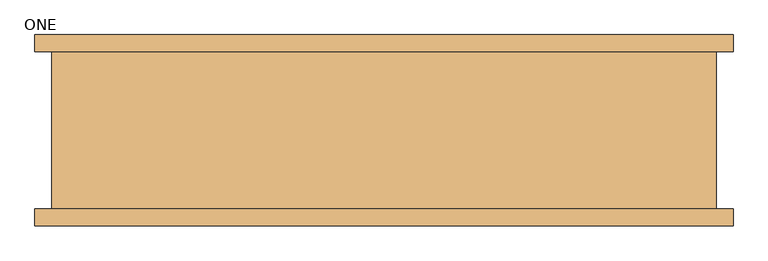
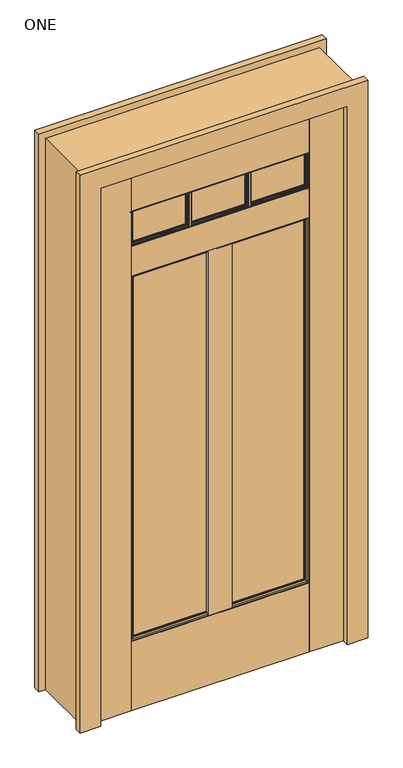
"""IFC4 building model written with IfcOpenShell, lengths in millimetres: door geometry, Door-Exterior-Simpson-Craftsman : ONE."""

from ifc_helpers import new_model, si_unit, point, frame, frame_2d, origin, origin_with_axes, place, context, project, spatial, polyline, circle_curve, ellipse_curve, trimmed, segment, composite_curve, outline, extrude, faceted_brep, source, transform, mapped, element, save
from ifc_brep_helpers import plane_surface, cylinder_surface, advanced_brep


def one_efa2d6c3(model_context):
    return source(origin(), model_context, "Body", "SolidModel", [
        extrude(outline(composite_curve([segment(polyline([(114.0354167, -78.5495), (114.0354167, -80.264), (116.1486027, -80.6366117)]), True, "CONTINUOUS"), segment(trimmed(circle_curve(frame_2d((115.7075363, -83.1380234)), 2.54), [point((116.1486027, -80.6366117))], [point((118.208948, -82.696957))], False, "CARTESIAN"), True, "CONTINUOUS"), segment(polyline([(118.208948, -82.696957), (118.7696182, -85.8766758), (120.0821906, -85.991511)]), True, "CONTINUOUS"), segment(trimmed(circle_curve(frame_2d((120.0157779, -86.7506113)), 0.762), [point((120.0821906, -85.991511))], [point((120.7662014, -86.6182914))], False, "CARTESIAN"), True, "CONTINUOUS"), segment(polyline([(120.7662014, -86.6182914), (121.1685282, -88.9), (98.9648051, -88.9), (99.3671319, -86.6182914)]), True, "CONTINUOUS"), segment(trimmed(circle_curve(frame_2d((100.1175554, -86.7506113)), 0.762), [point((99.3671319, -86.6182914))], [point((100.0511427, -85.991511))], False, "CARTESIAN"), True, "CONTINUOUS"), segment(polyline([(100.0511427, -85.991511), (101.3637152, -85.8766758), (101.9243854, -82.696957)]), True, "CONTINUOUS"), segment(trimmed(circle_curve(frame_2d((104.4257971, -83.1380234)), 2.54), [point((101.9243854, -82.696957))], [point((103.9847307, -80.6366117))], False, "CARTESIAN"), True, "CONTINUOUS"), segment(polyline([(103.9847307, -80.6366117), (106.0979167, -80.264), (106.0979167, -78.5495), (114.0354167, -78.5495)]), True, "CONTINUOUS")], self_intersect=False)), frame((0.0, 0.0, 1817.6875), z_axis=(0.0, 0.0, 1.0), x_axis=(1.0, 0.0, 0.0)), (0.0, 0.0, 1.0), 139.7),
        extrude(outline(composite_curve([segment(polyline([(114.0354167, -118.3005), (106.0979167, -118.3005), (106.0979167, -116.586), (103.9847307, -116.2133883)]), True, "CONTINUOUS"), segment(trimmed(circle_curve(frame_2d((104.4257971, -113.7119766)), 2.54), [point((103.9847307, -116.2133883))], [point((101.9243854, -114.153043))], False, "CARTESIAN"), True, "CONTINUOUS"), segment(polyline([(101.9243854, -114.153043), (101.3637152, -110.9733242), (100.0511427, -110.858489)]), True, "CONTINUOUS"), segment(trimmed(circle_curve(frame_2d((100.1175554, -110.0993887)), 0.762), [point((100.0511427, -110.858489))], [point((99.3671319, -110.2317086))], False, "CARTESIAN"), True, "CONTINUOUS"), segment(polyline([(99.3671319, -110.2317086), (98.9648051, -107.95), (121.1685282, -107.95), (120.7662014, -110.2317086)]), True, "CONTINUOUS"), segment(trimmed(circle_curve(frame_2d((120.0157779, -110.0993887)), 0.762), [point((120.7662014, -110.2317086))], [point((120.0821906, -110.858489))], False, "CARTESIAN"), True, "CONTINUOUS"), segment(polyline([(120.0821906, -110.858489), (118.7696182, -110.9733242), (118.208948, -114.153043)]), True, "CONTINUOUS"), segment(trimmed(circle_curve(frame_2d((115.7075363, -113.7119766)), 2.54), [point((118.208948, -114.153043))], [point((116.1486027, -116.2133883))], False, "CARTESIAN"), True, "CONTINUOUS"), segment(polyline([(116.1486027, -116.2133883), (114.0354167, -116.586), (114.0354167, -118.3005)]), True, "CONTINUOUS")], self_intersect=False)), frame((0.0, 0.0, 1817.6875), z_axis=(0.0, 0.0, 1.0), x_axis=(1.0, 0.0, 0.0)), (0.0, 0.0, 1.0), 139.7),
        extrude(outline(composite_curve([segment(polyline([(-106.0979167, -78.5495), (-106.0979167, -80.264), (-103.9847307, -80.6366117)]), True, "CONTINUOUS"), segment(trimmed(circle_curve(frame_2d((-104.4257971, -83.1380234)), 2.54), [point((-103.9847307, -80.6366117))], [point((-101.9243854, -82.696957))], False, "CARTESIAN"), True, "CONTINUOUS"), segment(polyline([(-101.9243854, -82.696957), (-101.3637152, -85.8766758), (-100.0511427, -85.991511)]), True, "CONTINUOUS"), segment(trimmed(circle_curve(frame_2d((-100.1175554, -86.7506113)), 0.762), [point((-100.0511427, -85.991511))], [point((-99.3671319, -86.6182914))], False, "CARTESIAN"), True, "CONTINUOUS"), segment(polyline([(-99.3671319, -86.6182914), (-98.9648051, -88.9), (-121.1685282, -88.9), (-120.7662014, -86.6182914)]), True, "CONTINUOUS"), segment(trimmed(circle_curve(frame_2d((-120.0157779, -86.7506113)), 0.762), [point((-120.7662014, -86.6182914))], [point((-120.0821906, -85.991511))], False, "CARTESIAN"), True, "CONTINUOUS"), segment(polyline([(-120.0821906, -85.991511), (-118.7696182, -85.8766758), (-118.208948, -82.696957)]), True, "CONTINUOUS"), segment(trimmed(circle_curve(frame_2d((-115.7075363, -83.1380234)), 2.54), [point((-118.208948, -82.696957))], [point((-116.1486027, -80.6366117))], False, "CARTESIAN"), True, "CONTINUOUS"), segment(polyline([(-116.1486027, -80.6366117), (-114.0354167, -80.264), (-114.0354167, -78.5495), (-106.0979167, -78.5495)]), True, "CONTINUOUS")], self_intersect=False)), frame((0.0, 0.0, 1817.6875), z_axis=(0.0, 0.0, 1.0), x_axis=(1.0, 0.0, 0.0)), (0.0, 0.0, 1.0), 139.7),
        extrude(outline(composite_curve([segment(polyline([(-106.0979167, -118.3005), (-114.0354167, -118.3005), (-114.0354167, -116.586), (-116.1486027, -116.2133883)]), True, "CONTINUOUS"), segment(trimmed(circle_curve(frame_2d((-115.7075363, -113.7119766)), 2.54), [point((-116.1486027, -116.2133883))], [point((-118.208948, -114.153043))], False, "CARTESIAN"), True, "CONTINUOUS"), segment(polyline([(-118.208948, -114.153043), (-118.7696182, -110.9733242), (-120.0821906, -110.858489)]), True, "CONTINUOUS"), segment(trimmed(circle_curve(frame_2d((-120.0157779, -110.0993887)), 0.762), [point((-120.0821906, -110.858489))], [point((-120.7662014, -110.2317086))], False, "CARTESIAN"), True, "CONTINUOUS"), segment(polyline([(-120.7662014, -110.2317086), (-121.1685282, -107.95), (-98.9648051, -107.95), (-99.3671319, -110.2317086)]), True, "CONTINUOUS"), segment(trimmed(circle_curve(frame_2d((-100.1175554, -110.0993887)), 0.762), [point((-99.3671319, -110.2317086))], [point((-100.0511427, -110.858489))], False, "CARTESIAN"), True, "CONTINUOUS"), segment(polyline([(-100.0511427, -110.858489), (-101.3637152, -110.9733242), (-101.9243854, -114.153043)]), True, "CONTINUOUS"), segment(trimmed(circle_curve(frame_2d((-104.4257971, -113.7119766)), 2.54), [point((-101.9243854, -114.153043))], [point((-103.9847307, -116.2133883))], False, "CARTESIAN"), True, "CONTINUOUS"), segment(polyline([(-103.9847307, -116.2133883), (-106.0979167, -116.586), (-106.0979167, -118.3005)]), True, "CONTINUOUS")], self_intersect=False)), frame((0.0, 0.0, 1817.6875), z_axis=(0.0, 0.0, 1.0), x_axis=(1.0, 0.0, 0.0)), (0.0, 0.0, 1.0), 139.7),
        extrude(outline(polyline([(44.45, -78.7796875), (44.45, -118.0703125), (-44.45, -118.0703125), (-44.45, -78.7796875), (44.45, -78.7796875)])), frame((0.0, 0.0, 271.4625), z_axis=(0.0, 0.0, 1.0), x_axis=(1.0, 0.0, 0.0)), (0.0, 0.0, 1.0), 1431.925),
        extrude(outline(polyline([(419.89375, -78.7796875), (419.89375, -118.0703125), (330.99375, -118.0703125), (330.99375, -78.7796875), (419.89375, -78.7796875)])), frame((0.0, 0.0, 271.4625), z_axis=(0.0, 0.0, 1.0), x_axis=(1.0, 0.0, 0.0)), (0.0, 0.0, 1.0), 1431.925),
        extrude(outline(polyline([(-330.99375, -78.7796875), (-330.99375, -118.0703125), (-419.89375, -118.0703125), (-419.89375, -78.7796875), (-330.99375, -78.7796875)])), frame((0.0, 0.0, 271.4625), z_axis=(0.0, 0.0, 1.0), x_axis=(1.0, 0.0, 0.0)), (0.0, 0.0, 1.0), 1431.925),
        extrude(outline(polyline([(330.2, -107.95), (-330.2, -107.95), (-330.2, -88.9), (330.2, -88.9), (330.2, -107.95)])), frame((0.0, 0.0, 271.4625), z_axis=(0.0, 0.0, 1.0), x_axis=(1.0, 0.0, 0.0)), (0.0, 0.0, 1.0), 1431.925),
        extrude(outline(composite_curve([segment(polyline([(334.16875, -78.5495), (334.16875, -80.264), (336.281936, -80.6366117)]), True, "CONTINUOUS"), segment(trimmed(circle_curve(frame_2d((335.8408696, -83.1380234)), 2.54), [point((336.281936, -80.6366117))], [point((338.3422813, -82.696957))], False, "CARTESIAN"), True, "CONTINUOUS"), segment(polyline([(338.3422813, -82.696957), (338.9029515, -85.8766758), (340.2155239, -85.991511)]), True, "CONTINUOUS"), segment(trimmed(circle_curve(frame_2d((340.1491113, -86.7506113)), 0.762), [point((340.2155239, -85.991511))], [point((340.8995348, -86.6182914))], False, "CARTESIAN"), True, "CONTINUOUS"), segment(polyline([(340.8995348, -86.6182914), (341.3018616, -88.9), (319.0981384, -88.9), (319.5004652, -86.6182914)]), True, "CONTINUOUS"), segment(trimmed(circle_curve(frame_2d((320.2508887, -86.7506113)), 0.762), [point((319.5004652, -86.6182914))], [point((320.1844761, -85.991511))], False, "CARTESIAN"), True, "CONTINUOUS"), segment(polyline([(320.1844761, -85.991511), (321.4970485, -85.8766758), (322.0577187, -82.696957)]), True, "CONTINUOUS"), segment(trimmed(circle_curve(frame_2d((324.5591304, -83.1380234)), 2.54), [point((322.0577187, -82.696957))], [point((324.118064, -80.6366117))], False, "CARTESIAN"), True, "CONTINUOUS"), segment(polyline([(324.118064, -80.6366117), (326.23125, -80.264), (326.23125, -78.5495), (334.16875, -78.5495)]), True, "CONTINUOUS")], self_intersect=False)), frame((0.0, 0.0, 1817.6875), z_axis=(0.0, 0.0, 1.0), x_axis=(1.0, 0.0, 0.0)), (0.0, 0.0, 1.0), 139.7),
        extrude(outline(composite_curve([segment(polyline([(334.16875, -118.3005), (326.23125, -118.3005), (326.23125, -116.586), (324.118064, -116.2133883)]), True, "CONTINUOUS"), segment(trimmed(circle_curve(frame_2d((324.5591304, -113.7119766)), 2.54), [point((324.118064, -116.2133883))], [point((322.0577187, -114.153043))], False, "CARTESIAN"), True, "CONTINUOUS"), segment(polyline([(322.0577187, -114.153043), (321.4970485, -110.9733242), (320.1844761, -110.858489)]), True, "CONTINUOUS"), segment(trimmed(circle_curve(frame_2d((320.2508887, -110.0993887)), 0.762), [point((320.1844761, -110.858489))], [point((319.5004652, -110.2317086))], False, "CARTESIAN"), True, "CONTINUOUS"), segment(polyline([(319.5004652, -110.2317086), (319.0981384, -107.95), (341.3018616, -107.95), (340.8995348, -110.2317086)]), True, "CONTINUOUS"), segment(trimmed(circle_curve(frame_2d((340.1491113, -110.0993887)), 0.762), [point((340.8995348, -110.2317086))], [point((340.2155239, -110.858489))], False, "CARTESIAN"), True, "CONTINUOUS"), segment(polyline([(340.2155239, -110.858489), (338.9029515, -110.9733242), (338.3422813, -114.153043)]), True, "CONTINUOUS"), segment(trimmed(circle_curve(frame_2d((335.8408696, -113.7119766)), 2.54), [point((338.3422813, -114.153043))], [point((336.281936, -116.2133883))], False, "CARTESIAN"), True, "CONTINUOUS"), segment(polyline([(336.281936, -116.2133883), (334.16875, -116.586), (334.16875, -118.3005)]), True, "CONTINUOUS")], self_intersect=False)), frame((0.0, 0.0, 1817.6875), z_axis=(0.0, 0.0, 1.0), x_axis=(1.0, 0.0, 0.0)), (0.0, 0.0, 1.0), 139.7),
        extrude(outline(composite_curve([segment(polyline([(-78.5495, 1813.71875), (-80.264, 1813.71875), (-80.6366117, 1811.605564)]), True, "CONTINUOUS"), segment(trimmed(circle_curve(frame_2d((-83.1380234, 1812.0466304)), 2.54), [point((-80.6366117, 1811.605564))], [point((-82.696957, 1809.5452187))], False, "CARTESIAN"), True, "CONTINUOUS"), segment(polyline([(-82.696957, 1809.5452187), (-85.8766758, 1808.9845485), (-85.991511, 1807.6719761)]), True, "CONTINUOUS"), segment(trimmed(circle_curve(frame_2d((-86.7506113, 1807.7383887)), 0.762), [point((-85.991511, 1807.6719761))], [point((-86.6182914, 1806.9879652))], False, "CARTESIAN"), True, "CONTINUOUS"), segment(polyline([(-86.6182914, 1806.9879652), (-88.9, 1806.5856384), (-88.9, 1828.7893616), (-86.6182914, 1828.3870348)]), True, "CONTINUOUS"), segment(trimmed(circle_curve(frame_2d((-86.7506113, 1827.6366113)), 0.762), [point((-86.6182914, 1828.3870348))], [point((-85.991511, 1827.7030239))], False, "CARTESIAN"), True, "CONTINUOUS"), segment(polyline([(-85.991511, 1827.7030239), (-85.8766758, 1826.3904515), (-82.696957, 1825.8297813)]), True, "CONTINUOUS"), segment(trimmed(circle_curve(frame_2d((-83.1380234, 1823.3283696)), 2.54), [point((-82.696957, 1825.8297813))], [point((-80.6366117, 1823.769436))], False, "CARTESIAN"), True, "CONTINUOUS"), segment(polyline([(-80.6366117, 1823.769436), (-80.264, 1821.65625), (-78.5495, 1821.65625), (-78.5495, 1813.71875)]), True, "CONTINUOUS")], self_intersect=False)), frame((-330.2, 0.0, 0.0), z_axis=(1.0, 0.0, 0.0), x_axis=(0.0, 1.0, 0.0)), (0.0, 0.0, 1.0), 660.4),
        extrude(outline(composite_curve([segment(polyline([(-118.3005, 1813.71875), (-118.3005, 1821.65625), (-116.586, 1821.65625), (-116.2133883, 1823.769436)]), True, "CONTINUOUS"), segment(trimmed(circle_curve(frame_2d((-113.7119766, 1823.3283696)), 2.54), [point((-116.2133883, 1823.769436))], [point((-114.153043, 1825.8297813))], False, "CARTESIAN"), True, "CONTINUOUS"), segment(polyline([(-114.153043, 1825.8297813), (-110.9733242, 1826.3904515), (-110.858489, 1827.7030239)]), True, "CONTINUOUS"), segment(trimmed(circle_curve(frame_2d((-110.0993887, 1827.6366113)), 0.762), [point((-110.858489, 1827.7030239))], [point((-110.2317086, 1828.3870348))], False, "CARTESIAN"), True, "CONTINUOUS"), segment(polyline([(-110.2317086, 1828.3870348), (-107.95, 1828.7893616), (-107.95, 1806.5856384), (-110.2317086, 1806.9879652)]), True, "CONTINUOUS"), segment(trimmed(circle_curve(frame_2d((-110.0993887, 1807.7383887)), 0.762), [point((-110.2317086, 1806.9879652))], [point((-110.858489, 1807.6719761))], False, "CARTESIAN"), True, "CONTINUOUS"), segment(polyline([(-110.858489, 1807.6719761), (-110.9733242, 1808.9845485), (-114.153043, 1809.5452187)]), True, "CONTINUOUS"), segment(trimmed(circle_curve(frame_2d((-113.7119766, 1812.0466304)), 2.54), [point((-114.153043, 1809.5452187))], [point((-116.2133883, 1811.605564))], False, "CARTESIAN"), True, "CONTINUOUS"), segment(polyline([(-116.2133883, 1811.605564), (-116.586, 1813.71875), (-118.3005, 1813.71875)]), True, "CONTINUOUS")], self_intersect=False)), frame((-330.2, 0.0, 0.0), z_axis=(1.0, 0.0, 0.0), x_axis=(0.0, 1.0, 0.0)), (0.0, 0.0, 1.0), 660.4),
        extrude(outline(composite_curve([segment(polyline([(-78.5495, 1953.41875), (-80.264, 1953.41875), (-80.6366117, 1951.305564)]), True, "CONTINUOUS"), segment(trimmed(circle_curve(frame_2d((-83.1380234, 1951.7466304)), 2.54), [point((-80.6366117, 1951.305564))], [point((-82.696957, 1949.2452187))], False, "CARTESIAN"), True, "CONTINUOUS"), segment(polyline([(-82.696957, 1949.2452187), (-85.8766758, 1948.6845485), (-85.991511, 1947.3719761)]), True, "CONTINUOUS"), segment(trimmed(circle_curve(frame_2d((-86.7506113, 1947.4383887)), 0.762), [point((-85.991511, 1947.3719761))], [point((-86.6182914, 1946.6879652))], False, "CARTESIAN"), True, "CONTINUOUS"), segment(polyline([(-86.6182914, 1946.6879652), (-88.9, 1946.2856384), (-88.9, 1968.4893616), (-86.6182914, 1968.0870348)]), True, "CONTINUOUS"), segment(trimmed(circle_curve(frame_2d((-86.7506113, 1967.3366113)), 0.762), [point((-86.6182914, 1968.0870348))], [point((-85.991511, 1967.4030239))], False, "CARTESIAN"), True, "CONTINUOUS"), segment(polyline([(-85.991511, 1967.4030239), (-85.8766758, 1966.0904515), (-82.696957, 1965.5297813)]), True, "CONTINUOUS"), segment(trimmed(circle_curve(frame_2d((-83.1380234, 1963.0283696)), 2.54), [point((-82.696957, 1965.5297813))], [point((-80.6366117, 1963.469436))], False, "CARTESIAN"), True, "CONTINUOUS"), segment(polyline([(-80.6366117, 1963.469436), (-80.264, 1961.35625), (-78.5495, 1961.35625), (-78.5495, 1953.41875)]), True, "CONTINUOUS")], self_intersect=False)), frame((-330.2, 0.0, 0.0), z_axis=(1.0, 0.0, 0.0), x_axis=(0.0, 1.0, 0.0)), (0.0, 0.0, 1.0), 660.4),
        extrude(outline(composite_curve([segment(polyline([(-118.3005, 1953.41875), (-118.3005, 1961.35625), (-116.586, 1961.35625), (-116.2133883, 1963.469436)]), True, "CONTINUOUS"), segment(trimmed(circle_curve(frame_2d((-113.7119766, 1963.0283696)), 2.54), [point((-116.2133883, 1963.469436))], [point((-114.153043, 1965.5297813))], False, "CARTESIAN"), True, "CONTINUOUS"), segment(polyline([(-114.153043, 1965.5297813), (-110.9733242, 1966.0904515), (-110.858489, 1967.4030239)]), True, "CONTINUOUS"), segment(trimmed(circle_curve(frame_2d((-110.0993887, 1967.3366113)), 0.762), [point((-110.858489, 1967.4030239))], [point((-110.2317086, 1968.0870348))], False, "CARTESIAN"), True, "CONTINUOUS"), segment(polyline([(-110.2317086, 1968.0870348), (-107.95, 1968.4893616), (-107.95, 1946.2856384), (-110.2317086, 1946.6879652)]), True, "CONTINUOUS"), segment(trimmed(circle_curve(frame_2d((-110.0993887, 1947.4383887)), 0.762), [point((-110.2317086, 1946.6879652))], [point((-110.858489, 1947.3719761))], False, "CARTESIAN"), True, "CONTINUOUS"), segment(polyline([(-110.858489, 1947.3719761), (-110.9733242, 1948.6845485), (-114.153043, 1949.2452187)]), True, "CONTINUOUS"), segment(trimmed(circle_curve(frame_2d((-113.7119766, 1951.7466304)), 2.54), [point((-114.153043, 1949.2452187))], [point((-116.2133883, 1951.305564))], False, "CARTESIAN"), True, "CONTINUOUS"), segment(polyline([(-116.2133883, 1951.305564), (-116.586, 1953.41875), (-118.3005, 1953.41875)]), True, "CONTINUOUS")], self_intersect=False)), frame((-330.2, 0.0, 0.0), z_axis=(1.0, 0.0, 0.0), x_axis=(0.0, 1.0, 0.0)), (0.0, 0.0, 1.0), 660.4),
        extrude(outline(composite_curve([segment(polyline([(-326.23125, -78.5495), (-326.23125, -80.264), (-324.118064, -80.6366117)]), True, "CONTINUOUS"), segment(trimmed(circle_curve(frame_2d((-324.5591304, -83.1380234)), 2.54), [point((-324.118064, -80.6366117))], [point((-322.0577187, -82.696957))], False, "CARTESIAN"), True, "CONTINUOUS"), segment(polyline([(-322.0577187, -82.696957), (-321.4970485, -85.8766758), (-320.1844761, -85.991511)]), True, "CONTINUOUS"), segment(trimmed(circle_curve(frame_2d((-320.2508887, -86.7506113)), 0.762), [point((-320.1844761, -85.991511))], [point((-319.5004652, -86.6182914))], False, "CARTESIAN"), True, "CONTINUOUS"), segment(polyline([(-319.5004652, -86.6182914), (-319.0981384, -88.9), (-341.3018616, -88.9), (-340.8995348, -86.6182914)]), True, "CONTINUOUS"), segment(trimmed(circle_curve(frame_2d((-340.1491113, -86.7506113)), 0.762), [point((-340.8995348, -86.6182914))], [point((-340.2155239, -85.991511))], False, "CARTESIAN"), True, "CONTINUOUS"), segment(polyline([(-340.2155239, -85.991511), (-338.9029515, -85.8766758), (-338.3422813, -82.696957)]), True, "CONTINUOUS"), segment(trimmed(circle_curve(frame_2d((-335.8408696, -83.1380234)), 2.54), [point((-338.3422813, -82.696957))], [point((-336.281936, -80.6366117))], False, "CARTESIAN"), True, "CONTINUOUS"), segment(polyline([(-336.281936, -80.6366117), (-334.16875, -80.264), (-334.16875, -78.5495), (-326.23125, -78.5495)]), True, "CONTINUOUS")], self_intersect=False)), frame((0.0, 0.0, 1817.6875), z_axis=(0.0, 0.0, 1.0), x_axis=(1.0, 0.0, 0.0)), (0.0, 0.0, 1.0), 139.7),
        extrude(outline(composite_curve([segment(polyline([(-326.23125, -118.3005), (-334.16875, -118.3005), (-334.16875, -116.586), (-336.281936, -116.2133883)]), True, "CONTINUOUS"), segment(trimmed(circle_curve(frame_2d((-335.8408696, -113.7119766)), 2.54), [point((-336.281936, -116.2133883))], [point((-338.3422813, -114.153043))], False, "CARTESIAN"), True, "CONTINUOUS"), segment(polyline([(-338.3422813, -114.153043), (-338.9029515, -110.9733242), (-340.2155239, -110.858489)]), True, "CONTINUOUS"), segment(trimmed(circle_curve(frame_2d((-340.1491113, -110.0993887)), 0.762), [point((-340.2155239, -110.858489))], [point((-340.8995348, -110.2317086))], False, "CARTESIAN"), True, "CONTINUOUS"), segment(polyline([(-340.8995348, -110.2317086), (-341.3018616, -107.95), (-319.0981384, -107.95), (-319.5004652, -110.2317086)]), True, "CONTINUOUS"), segment(trimmed(circle_curve(frame_2d((-320.2508887, -110.0993887)), 0.762), [point((-319.5004652, -110.2317086))], [point((-320.1844761, -110.858489))], False, "CARTESIAN"), True, "CONTINUOUS"), segment(polyline([(-320.1844761, -110.858489), (-321.4970485, -110.9733242), (-322.0577187, -114.153043)]), True, "CONTINUOUS"), segment(trimmed(circle_curve(frame_2d((-324.5591304, -113.7119766)), 2.54), [point((-322.0577187, -114.153043))], [point((-324.118064, -116.2133883))], False, "CARTESIAN"), True, "CONTINUOUS"), segment(polyline([(-324.118064, -116.2133883), (-326.23125, -116.586), (-326.23125, -118.3005)]), True, "CONTINUOUS")], self_intersect=False)), frame((0.0, 0.0, 1817.6875), z_axis=(0.0, 0.0, 1.0), x_axis=(1.0, 0.0, 0.0)), (0.0, 0.0, 1.0), 139.7),
        extrude(outline(polyline([(-330.2, -76.2), (-330.2, -120.65), (-457.2, -120.65), (-457.2, -76.2), (-330.2, -76.2)])), origin_with_axes(), (0.0, 0.0, 1.0), 2108.2),
        extrude(outline(polyline([(457.2, -76.2), (457.2, -120.65), (330.2, -120.65), (330.2, -76.2), (457.2, -76.2)])), origin_with_axes(), (0.0, 0.0, 1.0), 2108.2),
        extrude(outline(polyline([(330.2, -88.9), (330.2, -107.95), (-330.2, -107.95), (-330.2, -88.9), (330.2, -88.9)])), frame((0.0, 0.0, 1817.6875), z_axis=(0.0, 0.0, 1.0), x_axis=(1.0, 0.0, 0.0)), (0.0, 0.0, 1.0), 139.7),
        extrude(outline(polyline([(330.2, -76.2), (330.2, -120.65), (-330.2, -120.65), (-330.2, -76.2), (330.2, -76.2)])), frame((0.0, 0.0, 1957.3875), z_axis=(0.0, 0.0, 1.0), x_axis=(1.0, 0.0, 0.0)), (0.0, 0.0, 1.0), 150.8125),
        extrude(outline(polyline([(330.2, -76.2), (330.2, -120.65), (-330.2, -120.65), (-330.2, -76.2), (330.2, -76.2)])), frame((0.0, 0.0, 1703.3875), z_axis=(0.0, 0.0, 1.0), x_axis=(1.0, 0.0, 0.0)), (0.0, 0.0, 1.0), 114.3),
        extrude(outline(polyline([(330.2, -76.2), (330.2, -120.65), (-330.2, -120.65), (-330.2, -76.2), (330.2, -76.2)])), origin_with_axes(), (0.0, 0.0, 1.0), 271.4625),
        advanced_brep(
        [(-317.7512275, -110.8215438, 283.9112725), (317.7512275, -110.8215438, 283.9112725), (317.5, -107.95, 284.1625), (-317.5, -107.95, 284.1625), (-319.4070341, -112.5663998, 282.2554659), (319.4070341, -112.5663998, 282.2554659), (-320.6823867, -112.7456389, 280.9801133), (320.6823867, -112.7456389, 280.9801133), (-324.4223446, -117.3099547, 277.2401554), (324.4223446, -117.3099547, 277.2401554), (-330.2, -118.1219512, 271.4625), (330.2, -118.1219512, 271.4625), (-330.2, -107.95, 271.4625), (330.2, -107.95, 271.4625), (317.7512275, -110.8215438, 1690.9387275), (317.5, -107.95, 1690.6875), (319.4070341, -112.5663998, 1692.5945341), (320.6823867, -112.7456389, 1693.8698867), (324.4223446, -117.3099547, 1697.6098446), (330.2, -118.1219512, 1703.3875), (330.2, -107.95, 1703.3875), (-317.7512275, -110.8215438, 1690.9387275), (-317.5, -107.95, 1690.6875), (-319.4070341, -112.5663998, 1692.5945341), (-320.6823867, -112.7456389, 1693.8698867), (-324.4223446, -117.3099547, 1697.6098446), (-330.2, -118.1219512, 1703.3875), (-330.2, -107.95, 1703.3875)],
        [
            (0, 1),
            (1, 2),
            (2, 3),
            (3, 0),
            (4, 5),
            (5, 1, ellipse_curve(frame((319.6759231, -110.6531547, 281.9865769), z_axis=(-0.7071067811865475, 0.0, -0.7071067811865475), x_axis=(-0.7071067811865476, 0.0, 0.7071067811865474)), 2.732328, 1.9320476)),
            (0, 4, ellipse_curve(frame((-319.6759231, -110.6531547, 281.9865769), z_axis=(0.7071067811865475, 0.0, -0.7071067811865475), x_axis=(-0.7071067811865476, 0.0, -0.7071067811865474)), 2.732328, 1.9320476)),
            (6, 7),
            (7, 5),
            (4, 6),
            (8, 9),
            (9, 7, ellipse_curve(frame((325.0281918, -112.9991278, 276.6343082), z_axis=(-0.7071067811865475, 0.0, -0.7071067811865475), x_axis=(-0.7071067811865476, 0.0, 0.7071067811865474)), 6.1563429, 4.3531918)),
            (6, 8, ellipse_curve(frame((-325.0281918, -112.9991278, 276.6343082), z_axis=(0.7071067811865475, 0.0, -0.7071067811865475), x_axis=(-0.7071067811865476, 0.0, -0.7071067811865474)), 6.1563429, 4.3531918)),
            (10, 11),
            (11, 9),
            (8, 10),
            (12, 13),
            (13, 11),
            (10, 12),
            (1, 14),
            (14, 15),
            (15, 2),
            (5, 16),
            (16, 14, ellipse_curve(frame((319.6759231, -110.6531547, 1692.8634231), z_axis=(0.7071067811865475, 0.0, -0.7071067811865475), x_axis=(-0.7071067811865474, 0.0, -0.7071067811865476)), 2.732328, 1.9320476)),
            (7, 17),
            (17, 16),
            (9, 18),
            (18, 17, ellipse_curve(frame((325.0281918, -112.9991278, 1698.2156918), z_axis=(0.7071067811865475, 0.0, -0.7071067811865475), x_axis=(-0.7071067811865474, 0.0, -0.7071067811865476)), 6.1563429, 4.3531918)),
            (11, 19),
            (19, 18),
            (13, 20),
            (20, 19),
            (14, 21),
            (21, 22),
            (22, 15),
            (16, 23),
            (23, 21, ellipse_curve(frame((-319.6759231, -110.6531547, 1692.8634231), z_axis=(0.7071067811865475, 0.0, 0.7071067811865475), x_axis=(0.7071067811865476, 0.0, -0.7071067811865474)), 2.732328, 1.9320476)),
            (17, 24),
            (24, 23),
            (18, 25),
            (25, 24, ellipse_curve(frame((-325.0281918, -112.9991278, 1698.2156918), z_axis=(0.7071067811865475, 0.0, 0.7071067811865475), x_axis=(0.7071067811865476, 0.0, -0.7071067811865474)), 6.1563429, 4.3531918)),
            (19, 26),
            (26, 25),
            (20, 27),
            (27, 26),
            (12, 27),
            (22, 3),
            (21, 0),
            (23, 4),
            (24, 6),
            (25, 8),
            (26, 10),
        ],
        [
            plane_surface(frame((-317.5, -107.95, 284.1625), z_axis=(0.0, -0.08715574274767325, 0.9961946980917442), x_axis=(1.0, 0.0, 0.0))),
            cylinder_surface(frame((-330.2, -110.6531547, 281.9865769), z_axis=(-1.0, 0.0, 0.0), x_axis=(0.0, 0.0, -1.0)), 1.9320476),
            plane_surface(frame((-319.4070341, -112.5663998, 282.2554659), z_axis=(0.0, -0.9902680687415722, 0.13917310096005198), x_axis=(1.0, 0.0, 0.0))),
            cylinder_surface(frame((-330.2, -112.9991278, 276.6343082), z_axis=(-1.0, 0.0, 0.0), x_axis=(0.0, 0.0, -1.0)), 4.3531918),
            plane_surface(frame((-324.4223446, -117.3099547, 277.2401554), z_axis=(0.0, -0.9902680687415724, 0.13917310096005153), x_axis=(1.0, 0.0, 0.0))),
            plane_surface(frame((-330.2, -118.1219512, 271.4625), z_axis=(0.0, 0.0, -1.0), x_axis=(1.0, 0.0, 0.0))),
            plane_surface(frame((317.5, -107.95, 284.1625), z_axis=(-0.9961946980917454, -0.08715574274765947, 0.0), x_axis=(0.0, 0.0, 1.0))),
            cylinder_surface(frame((319.6759231, -110.6531547, 271.4625), z_axis=(0.0, 0.0, -1.0), x_axis=(1.0, 0.0, 0.0)), 1.9320476),
            plane_surface(frame((319.4070341, -112.5663998, 282.2554659), z_axis=(-0.13917310096006566, -0.9902680687415704, 0.0), x_axis=(0.0, 0.0, 1.0))),
            cylinder_surface(frame((325.0281918, -112.9991278, 271.4625), z_axis=(0.0, 0.0, -1.0), x_axis=(1.0, 0.0, 0.0)), 4.3531918),
            plane_surface(frame((324.4223446, -117.3099547, 277.2401554), z_axis=(-0.13917310096006522, -0.9902680687415705, 0.0), x_axis=(0.0, 0.0, 1.0))),
            plane_surface(frame((330.2, -118.1219512, 271.4625), z_axis=(1.0, 0.0, 0.0), x_axis=(0.0, 0.0, 1.0))),
            plane_surface(frame((317.5, -107.95, 1690.6875), z_axis=(0.0, -0.08715574274764569, -0.9961946980917467), x_axis=(-1.0, 0.0, 0.0))),
            cylinder_surface(frame((330.2, -110.6531547, 1692.8634231), z_axis=(1.0, 0.0, 0.0), x_axis=(0.0, 0.0, 1.0)), 1.9320476),
            plane_surface(frame((319.4070341, -112.5663998, 1692.5945341), z_axis=(0.0, -0.9902680687415685, -0.13917310096007934), x_axis=(-1.0, 0.0, 0.0))),
            cylinder_surface(frame((330.2, -112.9991278, 1698.2156918), z_axis=(1.0, 0.0, 0.0), x_axis=(0.0, 0.0, 1.0)), 4.3531918),
            plane_surface(frame((324.4223446, -117.3099547, 1697.6098446), z_axis=(0.0, -0.9902680687415686, -0.1391731009600789), x_axis=(-1.0, 0.0, 0.0))),
            plane_surface(frame((330.2, -118.1219512, 1703.3875), z_axis=(0.0, 0.0, 1.0), x_axis=(-1.0, 0.0, 0.0))),
            plane_surface(frame((-330.2, -107.95, 1703.3875), z_axis=(0.0, 1.0, 0.0), x_axis=(0.0, 0.0, -1.0))),
            plane_surface(frame((-317.5, -107.95, 1690.6875), z_axis=(0.9961946980917454, -0.08715574274765947, 0.0), x_axis=(0.0, 0.0, -1.0))),
            cylinder_surface(frame((-319.6759231, -110.6531547, 1703.3875), z_axis=(0.0, 0.0, 1.0), x_axis=(-1.0, 0.0, 0.0)), 1.9320476),
            plane_surface(frame((-319.4070341, -112.5663998, 1692.5945341), z_axis=(0.13917310096006566, -0.9902680687415704, 0.0), x_axis=(0.0, 0.0, -1.0))),
            cylinder_surface(frame((-325.0281918, -112.9991278, 1703.3875), z_axis=(0.0, 0.0, 1.0), x_axis=(-1.0, 0.0, 0.0)), 4.3531918),
            plane_surface(frame((-324.4223446, -117.3099547, 1697.6098446), z_axis=(0.13917310096006522, -0.9902680687415705, 0.0), x_axis=(0.0, 0.0, -1.0))),
            plane_surface(frame((-330.2, -118.1219512, 1703.3875), z_axis=(-1.0, 0.0, 0.0), x_axis=(0.0, 0.0, -1.0))),
        ],
        [
            (0, [[1, 2, 3, 4]]),
            (1, [[5, 6, -1, 7]]),
            (2, [[8, 9, -5, 10]]),
            (3, [[11, 12, -8, 13]]),
            (4, [[14, 15, -11, 16]]),
            (5, [[17, 18, -14, 19]]),
            (6, [[20, 21, 22, -2]]),
            (7, [[23, 24, -20, -6]]),
            (8, [[25, 26, -23, -9]]),
            (9, [[27, 28, -25, -12]]),
            (10, [[29, 30, -27, -15]]),
            (11, [[31, 32, -29, -18]]),
            (12, [[33, 34, 35, -21]]),
            (13, [[36, 37, -33, -24]]),
            (14, [[38, 39, -36, -26]]),
            (15, [[40, 41, -38, -28]]),
            (16, [[42, 43, -40, -30]]),
            (17, [[44, 45, -42, -32]]),
            (18, [[-17, 46, -44, -31], [-3, -22, -35, 47]]),
            (19, [[48, -4, -47, -34]]),
            (20, [[49, -7, -48, -37]]),
            (21, [[50, -10, -49, -39]]),
            (22, [[51, -13, -50, -41]]),
            (23, [[52, -16, -51, -43]]),
            (24, [[-46, -19, -52, -45]]),
        ],
    ),
        advanced_brep(
        [(-317.5, -88.9, 284.1625), (317.5, -88.9, 284.1625), (317.7512275, -86.0284562, 283.9112725), (-317.7512275, -86.0284562, 283.9112725), (319.4070341, -84.2836002, 282.2554659), (-319.4070341, -84.2836002, 282.2554659), (320.6823867, -84.1043611, 280.9801133), (-320.6823867, -84.1043611, 280.9801133), (324.4223446, -79.5400453, 277.2401554), (-324.4223446, -79.5400453, 277.2401554), (330.2, -78.7280488, 271.4625), (-330.2, -78.7280488, 271.4625), (330.2, -88.9, 271.4625), (-330.2, -88.9, 271.4625), (317.5, -88.9, 1690.6875), (317.7512275, -86.0284562, 1690.9387275), (319.4070341, -84.2836002, 1692.5945341), (320.6823867, -84.1043611, 1693.8698867), (324.4223446, -79.5400453, 1697.6098446), (330.2, -78.7280488, 1703.3875), (330.2, -88.9, 1703.3875), (-317.5, -88.9, 1690.6875), (-317.7512275, -86.0284562, 1690.9387275), (-319.4070341, -84.2836002, 1692.5945341), (-320.6823867, -84.1043611, 1693.8698867), (-324.4223446, -79.5400453, 1697.6098446), (-330.2, -78.7280488, 1703.3875), (-330.2, -88.9, 1703.3875)],
        [
            (0, 1),
            (1, 2),
            (2, 3),
            (3, 0),
            (2, 4, ellipse_curve(frame((319.6759231, -86.1968453, 281.9865769), z_axis=(-0.7071067811865475, 0.0, -0.7071067811865475), x_axis=(-0.7071067811865476, 0.0, 0.7071067811865474)), 2.732328, 1.9320476)),
            (4, 5),
            (5, 3, ellipse_curve(frame((-319.6759231, -86.1968453, 281.9865769), z_axis=(0.7071067811865475, 0.0, -0.7071067811865475), x_axis=(-0.7071067811865476, 0.0, -0.7071067811865474)), 2.732328, 1.9320476)),
            (4, 6),
            (6, 7),
            (7, 5),
            (6, 8, ellipse_curve(frame((325.0281918, -83.8508722, 276.6343082), z_axis=(-0.7071067811865475, 0.0, -0.7071067811865475), x_axis=(-0.7071067811865476, 0.0, 0.7071067811865474)), 6.1563429, 4.3531918)),
            (8, 9),
            (9, 7, ellipse_curve(frame((-325.0281918, -83.8508722, 276.6343082), z_axis=(0.7071067811865475, 0.0, -0.7071067811865475), x_axis=(-0.7071067811865476, 0.0, -0.7071067811865474)), 6.1563429, 4.3531918)),
            (8, 10),
            (10, 11),
            (11, 9),
            (10, 12),
            (12, 13),
            (13, 11),
            (1, 14),
            (14, 15),
            (15, 2),
            (15, 16, ellipse_curve(frame((319.6759231, -86.1968453, 1692.8634231), z_axis=(0.7071067811865475, 0.0, -0.7071067811865475), x_axis=(-0.7071067811865474, 0.0, -0.7071067811865476)), 2.732328, 1.9320476)),
            (16, 4),
            (16, 17),
            (17, 6),
            (17, 18, ellipse_curve(frame((325.0281918, -83.8508722, 1698.2156918), z_axis=(0.7071067811865475, 0.0, -0.7071067811865475), x_axis=(-0.7071067811865474, 0.0, -0.7071067811865476)), 6.1563429, 4.3531918)),
            (18, 8),
            (18, 19),
            (19, 10),
            (19, 20),
            (20, 12),
            (14, 21),
            (21, 22),
            (22, 15),
            (22, 23, ellipse_curve(frame((-319.6759231, -86.1968453, 1692.8634231), z_axis=(0.7071067811865475, 0.0, 0.7071067811865475), x_axis=(0.7071067811865476, 0.0, -0.7071067811865474)), 2.732328, 1.9320476)),
            (23, 16),
            (23, 24),
            (24, 17),
            (24, 25, ellipse_curve(frame((-325.0281918, -83.8508722, 1698.2156918), z_axis=(0.7071067811865475, 0.0, 0.7071067811865475), x_axis=(0.7071067811865476, 0.0, -0.7071067811865474)), 6.1563429, 4.3531918)),
            (25, 18),
            (25, 26),
            (26, 19),
            (26, 27),
            (27, 20),
            (27, 13),
            (0, 21),
            (3, 22),
            (5, 23),
            (7, 24),
            (9, 25),
            (11, 26),
        ],
        [
            plane_surface(frame((-317.7512275, -86.0284562, 283.9112725), z_axis=(0.0, 0.08715574274767325, 0.9961946980917442), x_axis=(1.0, 0.0, 0.0))),
            cylinder_surface(frame((-330.2, -86.1968453, 281.9865769), z_axis=(-1.0, 0.0, 0.0), x_axis=(0.0, 0.0, -1.0)), 1.9320476),
            plane_surface(frame((-320.6823867, -84.1043611, 280.9801133), z_axis=(0.0, 0.9902680687415722, 0.13917310096005198), x_axis=(1.0, 0.0, 0.0))),
            cylinder_surface(frame((-330.2, -83.8508722, 276.6343082), z_axis=(-1.0, 0.0, 0.0), x_axis=(0.0, 0.0, -1.0)), 4.3531918),
            plane_surface(frame((-330.2, -78.7280488, 271.4625), z_axis=(0.0, 0.9902680687415724, 0.13917310096005153), x_axis=(1.0, 0.0, 0.0))),
            plane_surface(frame((-330.2, -88.9, 271.4625), z_axis=(0.0, 0.0, -1.0), x_axis=(1.0, 0.0, 0.0))),
            plane_surface(frame((317.7512275, -86.0284562, 283.9112725), z_axis=(-0.9961946980917454, 0.08715574274765947, 0.0), x_axis=(0.0, 0.0, 1.0))),
            cylinder_surface(frame((319.6759231, -86.1968453, 271.4625), z_axis=(0.0, 0.0, -1.0), x_axis=(1.0, 0.0, 0.0)), 1.9320476),
            plane_surface(frame((320.6823867, -84.1043611, 280.9801133), z_axis=(-0.13917310096006566, 0.9902680687415704, 0.0), x_axis=(0.0, 0.0, 1.0))),
            cylinder_surface(frame((325.0281918, -83.8508722, 271.4625), z_axis=(0.0, 0.0, -1.0), x_axis=(1.0, 0.0, 0.0)), 4.3531918),
            plane_surface(frame((330.2, -78.7280488, 271.4625), z_axis=(-0.13917310096006522, 0.9902680687415705, 0.0), x_axis=(0.0, 0.0, 1.0))),
            plane_surface(frame((330.2, -88.9, 271.4625), z_axis=(1.0, 0.0, 0.0), x_axis=(0.0, 0.0, 1.0))),
            plane_surface(frame((317.7512275, -86.0284562, 1690.9387275), z_axis=(0.0, 0.08715574274764569, -0.9961946980917467), x_axis=(-1.0, 0.0, 0.0))),
            cylinder_surface(frame((330.2, -86.1968453, 1692.8634231), z_axis=(1.0, 0.0, 0.0), x_axis=(0.0, 0.0, 1.0)), 1.9320476),
            plane_surface(frame((320.6823867, -84.1043611, 1693.8698867), z_axis=(0.0, 0.9902680687415685, -0.13917310096007934), x_axis=(-1.0, 0.0, 0.0))),
            cylinder_surface(frame((330.2, -83.8508722, 1698.2156918), z_axis=(1.0, 0.0, 0.0), x_axis=(0.0, 0.0, 1.0)), 4.3531918),
            plane_surface(frame((330.2, -78.7280488, 1703.3875), z_axis=(0.0, 0.9902680687415686, -0.1391731009600789), x_axis=(-1.0, 0.0, 0.0))),
            plane_surface(frame((330.2, -88.9, 1703.3875), z_axis=(0.0, 0.0, 1.0), x_axis=(-1.0, 0.0, 0.0))),
            plane_surface(frame((-317.5, -88.9, 1690.6875), z_axis=(0.0, -1.0, 0.0), x_axis=(0.0, 0.0, -1.0))),
            plane_surface(frame((-317.7512275, -86.0284562, 1690.9387275), z_axis=(0.9961946980917454, 0.08715574274765947, 0.0), x_axis=(0.0, 0.0, -1.0))),
            cylinder_surface(frame((-319.6759231, -86.1968453, 1703.3875), z_axis=(0.0, 0.0, 1.0), x_axis=(-1.0, 0.0, 0.0)), 1.9320476),
            plane_surface(frame((-320.6823867, -84.1043611, 1693.8698867), z_axis=(0.13917310096006566, 0.9902680687415704, 0.0), x_axis=(0.0, 0.0, -1.0))),
            cylinder_surface(frame((-325.0281918, -83.8508722, 1703.3875), z_axis=(0.0, 0.0, 1.0), x_axis=(-1.0, 0.0, 0.0)), 4.3531918),
            plane_surface(frame((-330.2, -78.7280488, 1703.3875), z_axis=(0.13917310096006522, 0.9902680687415705, 0.0), x_axis=(0.0, 0.0, -1.0))),
            plane_surface(frame((-330.2, -88.9, 1703.3875), z_axis=(-1.0, 0.0, 0.0), x_axis=(0.0, 0.0, -1.0))),
        ],
        [
            (0, [[1, 2, 3, 4]]),
            (1, [[-3, 5, 6, 7]]),
            (2, [[-6, 8, 9, 10]]),
            (3, [[-9, 11, 12, 13]]),
            (4, [[-12, 14, 15, 16]]),
            (5, [[-15, 17, 18, 19]]),
            (6, [[20, 21, 22, -2]]),
            (7, [[-22, 23, 24, -5]]),
            (8, [[-24, 25, 26, -8]]),
            (9, [[-26, 27, 28, -11]]),
            (10, [[-28, 29, 30, -14]]),
            (11, [[-30, 31, 32, -17]]),
            (12, [[33, 34, 35, -21]]),
            (13, [[-35, 36, 37, -23]]),
            (14, [[-37, 38, 39, -25]]),
            (15, [[-39, 40, 41, -27]]),
            (16, [[-41, 42, 43, -29]]),
            (17, [[-43, 44, 45, -31]]),
            (18, [[-18, -32, -45, 46], [-1, 47, -33, -20]]),
            (19, [[-47, -4, 48, -34]]),
            (20, [[-48, -7, 49, -36]]),
            (21, [[-49, -10, 50, -38]]),
            (22, [[-50, -13, 51, -40]]),
            (23, [[-51, -16, 52, -42]]),
            (24, [[-52, -19, -46, -44]]),
        ],
    ),
        faceted_brep([(457.2, -146.05, 2108.2), (457.2, -146.05, 0.0), (533.4, -146.05, 0.0), (533.4, -146.05, 2184.4), (-533.4, -146.05, 2184.4), (-533.4, -146.05, 0.0), (-457.2, -146.05, 0.0), (-457.2, -146.05, 2108.2), (533.4, -120.65, 0.0), (508.0, -120.65, 0.0), (508.0, -120.65, 2159.0), (-508.0, -120.65, 2159.0), (-508.0, -120.65, 0.0), (-533.4, -120.65, 0.0), (-533.4, -120.65, 2184.4), (533.4, -120.65, 2184.4), (-457.2, 146.05, 2108.2), (457.2, 146.05, 2108.2), (-457.2, 146.05, 0.0), (-508.0, 120.65, 0.0), (-533.4, 120.65, 0.0), (-533.4, 146.05, 0.0), (457.2, 146.05, 0.0), (533.4, 146.05, 0.0), (533.4, 120.65, 0.0), (508.0, 120.65, 0.0), (-508.0, 120.65, 2159.0), (508.0, 120.65, 2159.0), (-533.4, 146.05, 2184.4), (533.4, 146.05, 2184.4), (533.4, 120.65, 2184.4), (-533.4, 120.65, 2184.4)], [[[0, 1, 2, 3, 4, 5, 6, 7]], [[8, 9, 10, 11, 12, 13, 14, 15]], [[7, 16, 17, 0]], [[6, 18, 16, 7]], [[5, 13, 12, 19, 20, 21, 18, 6]], [[4, 14, 13, 5]], [[3, 15, 14, 4]], [[2, 8, 15, 3]], [[1, 22, 23, 24, 25, 9, 8, 2]], [[17, 22, 1, 0]], [[12, 11, 26, 19]], [[11, 10, 27, 26]], [[10, 9, 25, 27]], [[17, 16, 18, 21, 28, 29, 23, 22]], [[20, 19, 26, 27, 25, 24, 30, 31]], [[29, 30, 24, 23]], [[28, 31, 30, 29]], [[21, 20, 31, 28]]]),
    ])


if __name__ == "__main__":
    model = new_model("IFC4")
    model_context = context("Model", 3, world=origin())
    ifc_project = project(units=[si_unit("LENGTHUNIT", "METRE", prefix="MILLI")], contexts=[model_context])
    site = spatial("IfcSite", under=ifc_project)
    building = spatial("IfcBuilding", under=site)
    placement = place(None, origin())
    one_shape = one_efa2d6c3(model_context)
    element("IfcDoor", 1, ObjectType="Door-Exterior-Simpson-Craftsman : ONE", at=placement, inside=building, context=model_context, shape_type="MappedRepresentation", body=[
        mapped(one_shape, transform((0.0, 0.0, 0.0), x_axis=(1.0, 0.0, 0.0), y_axis=(0.0, 1.0, 0.0), z_axis=(0.0, 0.0, 1.0))),
    ])
    save(model, "model.ifc")

# Revit data of these elements
# Type "Door-Exterior-Simpson-Craftsman : ONE"
#   Type Mark = "D7"
#   Wood Species Note = "Available in Any Wood Species"
#   Wood Species = "http://simpsondoor.com/e-catalog/#10"
#   WaterBarrier Note = "This Door Comes with The Option of WaterBarrier with UltraBlock Technology. It is Turn Off as a Default"
#   UltraBlock Note = "This Door Comes with The Option of UltraBlock Technology. It is Turn On as a Default"
#   URL = "http://www.simpsondoor.com/"
#   SubSeries = "Palomar"
#   Product Page URL = "http://www.simpsondoor.com/door-products/exterior/craftsman-collection/"
#   Product Documentation Link = "http://www.simpsondoor.com/door-products/search/detail/?BaseSpecificationID=1491"
#   Notes = "Dozens of glass textures and colors are available. For a list of standard options visit the Simpson web site or submit a custom glass request."
#   Model = "6933"
#   Manufacturer = "Simpson Door Company"
#   Description = "Palomar II Two Panel - Three Lite"
#   Assembly Code = "B2020100"
#   Analytic Construction = "<None>"
#   Window Height = 0' - 10"
#   Top Rail Height = 0' - 5 15/16"
#   Thickness = 0' - 1 3/4"
#   Rough Width = 3' - 6"
#   Rough Height = 7' - 2"
#   Panel Thickness = 0' - 0 3/4"
#   Panel Stile Width = 0' - 5"
#   Panel Divider Width = 0' - 3 1/2"
#   Lock Rail Height = 0' - 7 3/8"
#   Height = 6' - 11"
#   Frame Width = 0' - 3"
#   Default Sill Height = 0' - 0"
#   Width = 3' - 0"
#   Bottom Rail Height = 0' - 10 11/16"
#   Bottom Panel Height = 4' - 8 3/8"
#   WaterBarrier with UltraBlock Technology = no
#   UltraBlock Option = yes
#   Show Frame [instance default] = yes
#   Number of Vertical Muntins = 2
#   Number of Panel Dividers = 1
#   Function = 1
#   Wall Closure = 3
#   Panel = 1X WOOD COMPOSITE TRIM
#   Glass = Glass - Simpson Doors - Clear
#   Frame = 1X WOOD COMPOSITE TRIM
# Element 1 (IfcDoor, "Door-Exterior-Simpson-Craftsman : ONE")
#   Materials on its faces: "1X WOOD COMPOSITE TRIM", "Glass - Simpson Doors - Clear"
# Materials
#   "1X WOOD COMPOSITE TRIM": class "Generic", colour RGB 88 61 61, transparency 0, Cost = 0
#   "Glass - Simpson Doors - Clear": class "Glass", colour RGB 0 0 255, transparency 0.75
